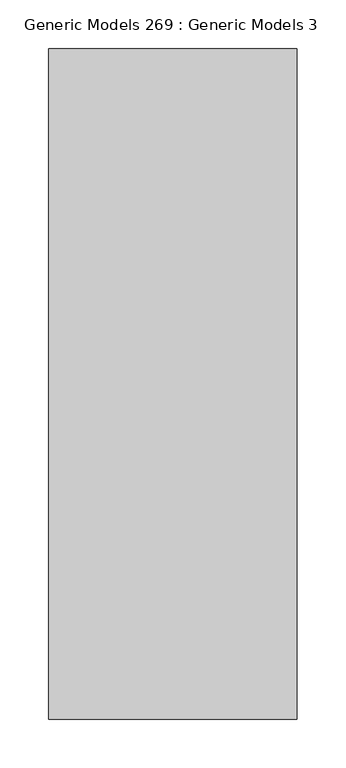
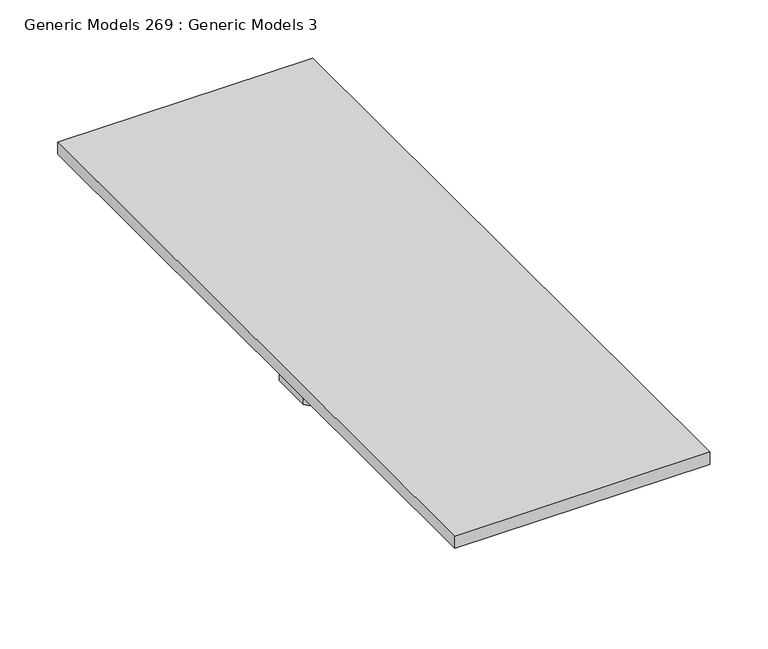
"""IFC4 building model written with IfcOpenShell, lengths in millimetres: proxy geometry, Generic Models 269 : Generic Models 3."""

from ifc_helpers import new_model, si_unit, frame, origin, place, context, project, spatial, polyline, outline, extrude, source, transform, mapped, element, save


def generic_models_269_generic_models_3_a750ed91(model_context):
    return source(origin(), model_context, "Body", "SweptSolid", [
        extrude(outline(polyline([(126739.396, 165.2002941), (126739.396, -88.337964), (126731.6836145, -88.337964), (126694.4947194, -20.1963119), (126694.4947194, 120.2990135), (126739.396, 165.2002941)])), frame((0.0, 662.7539193, 0.0), z_axis=(0.0, 1.0, 0.0), x_axis=(0.0, 0.0, 1.0)), (0.0, 0.0, 1.0), 41.7770469),
        extrude(outline(polyline([(-89.0736296, 1085.2769662), (164.9263704, 1085.2769662), (164.9263704, 399.7309662), (-89.0736296, 399.7309662), (-89.0736296, 1085.2769662)])), frame((0.0, 0.0, 126739.396), z_axis=(0.0, 0.0, 1.0), x_axis=(1.0, 0.0, 0.0)), (0.0, 0.0, 1.0), 12.7),
    ])


if __name__ == "__main__":
    model = new_model("IFC4")
    model_context = context("Model", 3, world=origin())
    ifc_project = project(units=[si_unit("LENGTHUNIT", "METRE", prefix="MILLI")], contexts=[model_context])
    site = spatial("IfcSite", under=ifc_project)
    building = spatial("IfcBuilding", under=site)
    placement = place(None, origin())
    generic_models_269_generic_models_3_shape = generic_models_269_generic_models_3_a750ed91(model_context)
    element("IfcBuildingElementProxy", 1, Name="Generic Models 269 : Generic Models 3", ObjectType="Generic Models 269 : Generic Models 3", at=placement, inside=building, context=model_context, shape_type="MappedRepresentation", body=[
        mapped(generic_models_269_generic_models_3_shape, transform((0.0, 0.0, 0.0), x_axis=(1.0, 0.0, 0.0), y_axis=(0.0, 1.0, 0.0), z_axis=(0.0, 0.0, 1.0))),
    ])
    save(model, "model.ifc")

# Revit data of these elements
# Element 1 (IfcBuildingElementProxy, "Generic Models 269 : Generic Models 3")
#   Materials on its faces: "_SHAPED \"T\" TREAD SUPPORT PER STRUCTURAL, PAINTED"
# Materials
#   "_SHAPED \"T\" TREAD SUPPORT PER STRUCTURAL, PAINTED": class "Metal", colour RGB 199 199 199, transparency 0, Description = "Structural steel 50ksi", Cost = 0
